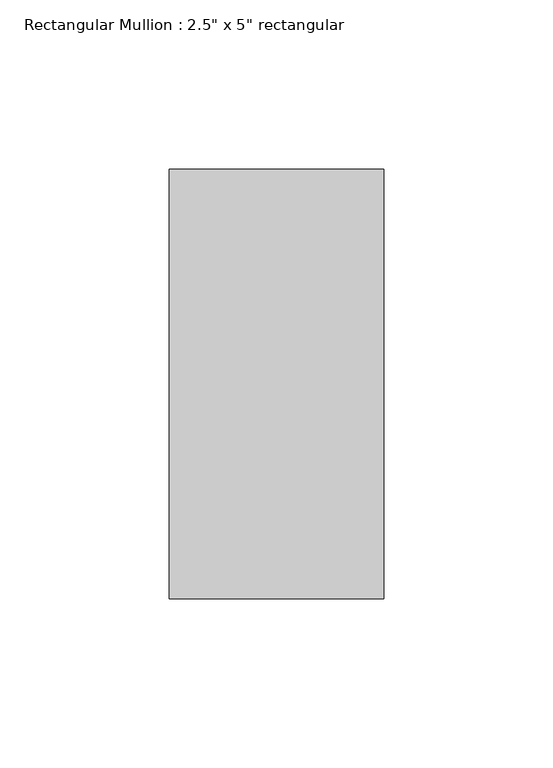
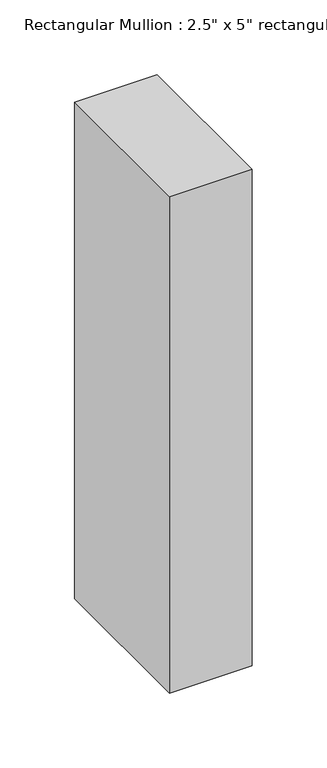
"""IFC4 building model written with IfcOpenShell, lengths in millimetres: member geometry."""

import ifcopenshell
import ifcopenshell.guid

model = None  # the IFC model being written
_history = None  # IfcOwnerHistory: only IFC2X3 demands one
_inside = {}  # id of a spatial element -> (the spatial element, [elements in it])
_under = {}  # id of a project, library or spatial element -> (it, [spatial elements below it])
_declared = {}  # id of a project -> (the project, [libraries it declares])
_typed = {}  # id of a type object -> (the type object, [elements of that type])
_made_of = {}  # id of a material, layer set ... -> (it, [elements and type objects made of it])


def new_model(schema):
    """Start an empty IFC model of exactly this schema.

    Asked for "IFC4X3", IfcOpenShell would pick the latest addendum, in which some entities
    have other attributes; the version numbers below select the first issue.
    IFC2X3 requires an IfcOwnerHistory on every rooted entity: one is made here for all.
    """
    global model, _history
    if schema == "IFC4X3":
        model = ifcopenshell.file(schema_version=(4, 3, 0, 0))
    else:
        model = ifcopenshell.file(schema=schema)
    _inside.clear()
    _under.clear()
    _declared.clear()
    _typed.clear()
    _made_of.clear()
    _history = None
    if model.schema == "IFC2X3":
        org = make("IfcOrganization", Name="unknown")
        user = make(
            "IfcPersonAndOrganization",
            ThePerson=make("IfcPerson", FamilyName="unknown"),
            TheOrganization=org,
        )
        app = make(
            "IfcApplication",
            ApplicationDeveloper=org,
            Version="unknown",
            ApplicationFullName="unknown",
            ApplicationIdentifier="unknown",
        )
        _history = make(
            "IfcOwnerHistory",
            OwningUser=user,
            OwningApplication=app,
            ChangeAction="ADDED",
            CreationDate=0,
        )
    return model


def make(cls, **values):
    """One entity of the class cls with the attributes given. An attribute that is None is left unset."""
    return model.create_entity(
        cls, **{name: value for name, value in values.items() if value is not None}
    )


def rooted(cls, **values):
    """An entity with a GlobalId (a new one), such as an element, a storey or a relation."""
    return make(cls, GlobalId=ifcopenshell.guid.new(), OwnerHistory=_history, **values)


def si_unit(unit_type, name, prefix=None):
    """IfcSIUnit, for example si_unit("LENGTHUNIT", "METRE", prefix="MILLI")."""
    return make("IfcSIUnit", UnitType=unit_type, Prefix=prefix, Name=name)


def assignment(units):
    """IfcUnitAssignment: the units of a project."""
    return None if units is None else make("IfcUnitAssignment", Units=units)


def point(xyz):
    """IfcCartesianPoint."""
    return None if xyz is None else make("IfcCartesianPoint", Coordinates=xyz)


def direction(xyz):
    """IfcDirection."""
    return None if xyz is None else make("IfcDirection", DirectionRatios=xyz)


def frame(location, z_axis=None, x_axis=None):
    """IfcAxis2Placement3D, a coordinate frame: its origin and axes. An axis left out is left unset."""
    return make(
        "IfcAxis2Placement3D",
        Location=point(location),
        Axis=direction(z_axis),
        RefDirection=direction(x_axis),
    )


def origin():
    """The frame at (0, 0, 0) with its axes left unset."""
    return frame((0.0, 0.0, 0.0))


def place(relative_to, where):
    """IfcLocalPlacement: puts the frame where relative to a parent placement (None: the world)."""
    return make(
        "IfcLocalPlacement", PlacementRelTo=relative_to, RelativePlacement=where
    )


def context(
    kind, dimensions, precision=None, world=None, true_north=None, identifier=None
):
    """IfcGeometricRepresentationContext, for example the 3D "Model" context."""
    return make(
        "IfcGeometricRepresentationContext",
        ContextIdentifier=identifier,
        ContextType=kind,
        CoordinateSpaceDimension=dimensions,
        Precision=precision,
        WorldCoordinateSystem=world,
        TrueNorth=true_north,
    )


def project(units=None, contexts=None):
    """IfcProject with its units and contexts."""
    return rooted(
        "IfcProject",
        Name="project",
        RepresentationContexts=contexts,
        UnitsInContext=assignment(units),
    )


def spatial(cls, under=None, at=None, **own):
    """A site, building, storey or space (cls), placed at a placement, below another one or the project."""
    s = rooted(cls, ObjectPlacement=at, **own)
    if under is not None:
        _under.setdefault(under.id(), (under, []))[1].append(s)
    return s


def polyline(points):
    """IfcPolyline through the points."""
    return make("IfcPolyline", Points=[point(p) for p in points])


def outline(outer, holes=None, kind="AREA"):
    """IfcArbitraryClosedProfileDef: a profile drawn as a closed curve; with holes, ...WithVoids."""
    if holes is None:
        return make("IfcArbitraryClosedProfileDef", ProfileType=kind, OuterCurve=outer)
    return make(
        "IfcArbitraryProfileDefWithVoids",
        ProfileType=kind,
        OuterCurve=outer,
        InnerCurves=holes,
    )


def extrude(swept, where, along, depth):
    """IfcExtrudedAreaSolid: the profile swept, set in the frame where, extruded along a direction by depth."""
    return make(
        "IfcExtrudedAreaSolid",
        SweptArea=swept,
        Position=where,
        ExtrudedDirection=direction(along),
        Depth=depth,
    )


def shape(context_of_items, identifier, shape_type, items):
    """IfcShapeRepresentation: the items that make up one representation, for example the "Body"."""
    return make(
        "IfcShapeRepresentation",
        ContextOfItems=context_of_items,
        RepresentationIdentifier=identifier,
        RepresentationType=shape_type,
        Items=items,
    )


def source(mapping_origin, context_of_items, identifier, shape_type, items):
    """IfcRepresentationMap: a shape defined once, which mapped items show again and again."""
    return make(
        "IfcRepresentationMap",
        MappingOrigin=mapping_origin,
        MappedRepresentation=shape(context_of_items, identifier, shape_type, items),
    )


def transform(
    local_origin,
    x_axis=None,
    y_axis=None,
    z_axis=None,
    scale=None,
    scale2=None,
    scale3=None,
    uniform=True,
):
    """IfcCartesianTransformationOperator3D, or its non-uniform kind. x_axis, y_axis, z_axis: its Axis1, 2, 3."""
    if uniform:
        return make(
            "IfcCartesianTransformationOperator3D",
            Axis1=direction(x_axis),
            Axis2=direction(y_axis),
            LocalOrigin=point(local_origin),
            Scale=scale,
            Axis3=direction(z_axis),
        )
    return make(
        "IfcCartesianTransformationOperator3DnonUniform",
        Axis1=direction(x_axis),
        Axis2=direction(y_axis),
        LocalOrigin=point(local_origin),
        Scale=scale,
        Axis3=direction(z_axis),
        Scale2=scale2,
        Scale3=scale3,
    )


def mapped(mapping_source, mapping_target):
    """IfcMappedItem: shows the shape of a source again, moved by a transform."""
    return make(
        "IfcMappedItem", MappingSource=mapping_source, MappingTarget=mapping_target
    )


def made_of(thing, what):
    """Note that an element or type object is made of a material, layer set ...; save() writes the relation."""
    if what is not None:
        _made_of.setdefault(what.id(), (what, []))[1].append(thing)
    return thing


def element(
    cls,
    number,
    at=None,
    inside=None,
    cuts=None,
    type_object=None,
    material=None,
    context=None,
    identifier="Body",
    shape_type=None,
    held_by="IfcProductDefinitionShape",
    body=None,
    shapes=None,
    **own,
):
    """One element of the class cls, such as IfcWall. Its Tag is "e" and its number.

    at: its placement. inside: the storey or other place that contains it. cuts: it is an
    opening in that element (IfcRelVoidsElement). A single representation is given by context,
    identifier, shape_type and body (its items); several are given by shapes. held_by: the class
    of the entity that holds the representations. save() writes the other relations.
    """
    e = rooted(cls, Tag="e%d" % number, ObjectPlacement=at, **own)
    if body is not None:
        shapes = [shape(context, identifier, shape_type, body)]
    if shapes is not None:
        e.Representation = make(held_by, Representations=shapes)
    if inside is not None:
        _inside.setdefault(inside.id(), (inside, []))[1].append(e)
    if cuts is not None:
        rooted(
            "IfcRelVoidsElement", RelatingBuildingElement=cuts, RelatedOpeningElement=e
        )
    if type_object is not None:
        _typed.setdefault(type_object.id(), (type_object, []))[1].append(e)
    return made_of(e, material)


def aggregate(whole, parts):
    """IfcRelAggregates: a whole, such as a stair, and the parts it consists of."""
    return rooted("IfcRelAggregates", RelatingObject=whole, RelatedObjects=parts)


def save(model, path):
    """Write the relations noted so far, then the file.

    IfcRelAggregates (storeys below a building ...), IfcRelContainedInSpatialStructure (elements
    in a storey), IfcRelDefinesByType, IfcRelAssociatesMaterial and IfcRelDeclares: one each for
    every whole, place, type object, material and project.
    """
    for whole, parts in _under.values():
        aggregate(whole, parts)
    for where, things in _inside.values():
        rooted(
            "IfcRelContainedInSpatialStructure",
            RelatedElements=things,
            RelatingStructure=where,
        )
    for kind, things in _typed.values():
        rooted("IfcRelDefinesByType", RelatedObjects=things, RelatingType=kind)
    for what, things in _made_of.values():
        rooted("IfcRelAssociatesMaterial", RelatedObjects=things, RelatingMaterial=what)
    for by, libraries in _declared.values():
        rooted("IfcRelDeclares", RelatingContext=by, RelatedDefinitions=libraries)
    model.write(path)


def member_5908c209(model_context):
    return source(origin(), model_context, "Body", "SweptSolid", [
        extrude(outline(polyline([(0.0, 63.5), (0.0, -63.5), (-63.5, -63.5), (-63.5, 63.5), (0.0, 63.5)])), frame((0.0, 0.0, -404.75), z_axis=(0.0, 0.0, 1.0), x_axis=(1.0, 0.0, 0.0)), (0.0, 0.0, 1.0), 404.75),
    ])


if __name__ == "__main__":
    model = new_model("IFC4")
    model_context = context("Model", 3, world=origin())
    ifc_project = project(units=[si_unit("LENGTHUNIT", "METRE", prefix="MILLI")], contexts=[model_context])
    site = spatial("IfcSite", under=ifc_project)
    building = spatial("IfcBuilding", under=site)
    placement = place(None, origin())
    member_shape = member_5908c209(model_context)
    element("IfcMember", 1, ObjectType="Rectangular Mullion : 2.5\" x 5\" rectangular", at=placement, inside=building, context=model_context, shape_type="MappedRepresentation", body=[
        mapped(member_shape, transform((0.0, 0.0, 0.0), x_axis=(1.0, 0.0, 0.0), y_axis=(0.0, 1.0, 0.0), z_axis=(0.0, 0.0, 1.0))),
    ])
    save(model, "model.ifc")

# Revit data of these elements
# Type "Rectangular Mullion : 2.5\" x 5\" rectangular"
#   built-in parameter 1007304 = 0.416667 (stored number, unit not read)
#   built-in parameter 1007301 = 0.104167 (stored number, unit not read)
#   built-in parameter 1007300 = 0.104167 (stored number, unit not read)
# Element 1 (IfcMember, "Rectangular Mullion : 2.5\" x 5\" rectangular")
#   Materials on its faces: "Metal - Aluminum 2"
# Materials
#   "Metal - Aluminum 2": class "Metal", colour RGB 189 187 185, transparency 0
